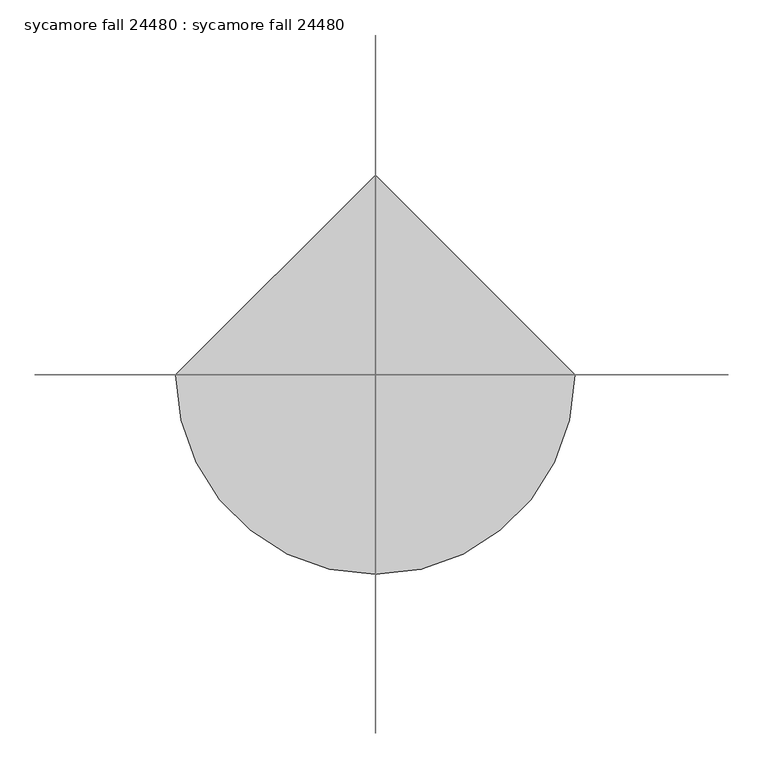
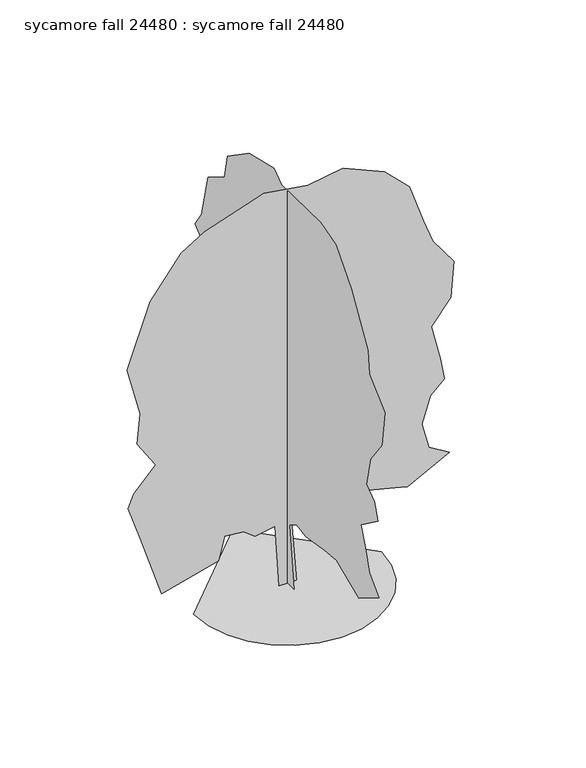
"""IFC4 building model written with IfcOpenShell, lengths in millimetres: proxy geometry, sycamore fall 24480 : sycamore fall 24480."""

from ifc_helpers import new_model, si_unit, origin, place, context, project, spatial, triangles, source, transform, mapped, element, save


def sycamore_fall_24480_sycamore_fall_24480_863b0ace(model_context):
    return source(origin(), model_context, "Body", "Tessellation", [
        triangles([(-350.832074, 1.54e-05, 0.0), (-519.2948653, -0.0002987, 2696.4612831), (-1365.6143188, -0.0002448, 2554.5769203), (-1847.3222706, -0.0002667, 2914.5200661), (-2641.8003754, -0.0002417, 2996.2572281), (-2887.1897575, -0.0001129, 2006.0772606), (-5273.8728561, 6.56e-05, 1384.1309212), (-6175.1399368, -0.000225, 4152.286084), (-6690.1497803, -0.000379, 5632.9271027), (-6446.9198593, -0.0004579, 6205.1631042), (-5531.3774872, -0.0006139, 7177.956633), (-6303.892543, -0.0007221, 8368.8851028), (-6175.1399368, -0.0008812, 9656.4100021), (-6722.3315369, -0.0011105, 11780.8123077), (-5756.700943, -0.001475, 14484.5891327), (-4453.1741135, -0.0017335, 16174.3476196), (-3471.3636932, -0.0018474, 16769.9263824), (-992.8925926, -0.0020555, 17606.8043701), (855.168877, -0.0021033, 17330.758429), (2322.4618732, -0.0021953, 17563.9046631), (4060.6175514, -0.0021804, 16802.108139), (5122.7937057, -0.0021041, 15772.114032), (5702.1926422, -0.001926, 14066.1495575), (6088.4498795, -0.0018163, 13003.948114), (6966.9590469, -0.0017145, 11827.7524658), (6860.9393555, -0.0015239, 10267.9906952), (6024.0607864, -0.0013645, 9237.9704269), (6413.7730453, -0.0011987, 7703.5832703), (6571.2529678, -0.001093, 6759.4920593), (5991.8790298, -0.0010025, 6212.3004593), (5637.8035492, -0.0008488, 5053.5531647), (5937.4468872, -0.0007297, 3944.5144638), (6794.2137772, -0.0007034, 3409.5910103), (5026.248436, -0.000519, 2510.7060516), (4511.2385925, -0.0005118, 2639.4635994), (2708.7041405, -0.0004867, 3090.0846405), (1446.8942413, -0.0004051, 2868.0127304), (1099.3210527, -0.0003972, 2929.1502777), (154.8209641, -0.0004225, 3487.5940979), (137.7651375, -0.0003627, 2991.9900467), (374.3524406, -1.63e-05, 0.0005208), (-4.19e-05, -473.1532413, 0.279514), (8.81e-05, -141.9955024, 2641.8259552), (4.65e-05, -654.9917061, 2992.6504715), (-2.36e-05, -1329.4982094, 2853.8647568), (-0.0001766, -2695.3944878, 3090.3639839), (-0.0002449, -3548.3255653, 3170.8058762), (-0.0004512, -5206.0293228, 2478.7960808), (-0.0005787, -6654.4885849, 3380.0506622), (-0.0004837, -5946.3626221, 4055.9948685), (-0.0004302, -5656.6756531, 4989.4437057), (-0.0003796, -5334.781929, 5826.3222748), (-0.0004627, -6557.9433151, 6727.5893555), (-0.0004219, -6332.6198593, 7435.7153183), (-0.0003424, -5721.0391663, 7854.179892), (-0.0003333, -6010.7261353, 9141.6792114), (-0.0003897, -6847.6297028, 10268.2697479), (-0.0003651, -7072.9275787, 11845.4560364), (-0.0002032, -5962.313974, 12858.9395233), (-0.0001885, -5849.7917725, 13873.2880737), (1.85e-05, -4658.8377228, 15836.7565979), (0.0001585, -3532.2727661, 17124.2814972), (0.0002908, -2408.9233109, 17446.1502228), (0.0005846, 426.8338666, 17381.7867096), (0.0006611, 989.4941082, 17779.9821716), (0.0008252, 2804.4619583, 17349.5793732), (0.0009496, 4340.6016243, 16287.3779297), (0.0009476, 4571.5633987, 15221.4429932), (0.0010368, 5770.0105957, 14484.8681854), (0.0010426, 6252.8386826, 12553.6069977), (0.0010659, 6703.459433, 11845.4560364), (0.0009883, 6168.8153229, 11394.8347046), (0.0009238, 6156.2678329, 9141.6792114), (0.0009203, 6220.656926, 8208.2303741), (0.0008056, 5448.1418701, 7146.0289307), (0.0008789, 6510.3433136, 6180.3977554), (0.0008979, 6703.459433, 5633.2061554), (0.0007283, 6027.5152267, 3219.1165901), (0.0006596, 5350.1995926, 2324.727578), (0.000618, 5264.7798065, 1458.5579189), (0.0004531, 3484.6733459, 1835.0388634), (0.0003699, 2840.9361855, 2156.9174721), (0.0003995, 2647.7947769, 3026.0004707), (0.0002502, 1392.4722725, 2446.6093826), (0.0002126, 1108.5996288, 2659.9106071), (0.0001468, 456.7626357, 2595.6741211), (6.52e-05, 395.9170037, 0.2796182), (-3939.7900429, -8e-07, 0.2427224), (-3835.6501785, -902.7404646, 0.2426104), (-3539.0037506, -1731.7626091, 0.2424986), (-3073.6507599, -2463.3147583, 0.2423909), (-2463.3147583, -3073.6507599, 0.2422916), (-1731.7626091, -3539.0037506, 0.242204), (-902.7404646, -3835.6501785, 0.2421326), (0.0001865, -3939.7900429, 0.2420805), (902.7404646, -3835.6501785, 0.2426061), (1731.7626091, -3539.0037506, 0.2426053), (2463.3147583, -3073.6507599, 0.2426287), (3073.6507599, -2463.3147583, 0.2426749), (3539.0037506, -1731.7626091, 0.2427417), (3835.6501785, -902.7404646, 0.2428276), (3939.7900429, 0.0003444, 0.242378), (-0.0005051, 3939.7900429, 0.2424674)], [[32, 33, 34], [41, 1, 2], [40, 41, 2], [6, 7, 8], [5, 6, 8], [32, 34, 35], [39, 40, 2], [31, 32, 35], [31, 35, 36], [28, 29, 30], [5, 8, 9], [5, 9, 10], [5, 10, 11], [4, 5, 11], [2, 3, 4], [39, 2, 4], [39, 4, 11], [24, 25, 26], [24, 26, 27], [30, 31, 36], [11, 12, 13], [39, 11, 13], [13, 14, 15], [39, 13, 15], [39, 15, 16], [39, 16, 17], [39, 17, 18], [39, 18, 19], [39, 19, 20], [39, 20, 21], [39, 21, 22], [39, 22, 23], [39, 23, 24], [39, 24, 27], [39, 27, 28], [39, 28, 30], [39, 30, 36], [39, 36, 37], [38, 39, 37], [48, 49, 50], [79, 80, 81], [86, 87, 42], [86, 42, 43], [47, 48, 50], [47, 50, 51], [70, 71, 72], [52, 53, 54], [52, 54, 55], [47, 51, 52], [83, 84, 85], [57, 58, 59], [56, 57, 59], [81, 82, 83], [79, 81, 83], [78, 79, 83], [77, 78, 83], [76, 77, 83], [75, 76, 83], [46, 47, 52], [64, 65, 66], [68, 69, 70], [66, 67, 68], [64, 66, 68], [75, 83, 85], [75, 85, 86], [75, 86, 43], [75, 43, 44], [73, 74, 75], [68, 70, 72], [64, 68, 72], [63, 64, 72], [63, 72, 73], [63, 73, 75], [63, 75, 44], [62, 63, 44], [61, 62, 44], [60, 61, 44], [59, 60, 44], [56, 59, 44], [55, 56, 44], [52, 55, 44], [46, 52, 44], [45, 46, 44], [102, 103, 88], [101, 102, 88], [101, 88, 89], [100, 101, 89], [100, 89, 90], [100, 90, 91], [99, 100, 91], [98, 99, 91], [98, 91, 92], [98, 92, 93], [98, 93, 94], [98, 94, 95], [98, 95, 96], [98, 96, 97]], closed=False),
    ])


if __name__ == "__main__":
    model = new_model("IFC4")
    model_context = context("Model", 3, world=origin())
    ifc_project = project(units=[si_unit("LENGTHUNIT", "METRE", prefix="MILLI")], contexts=[model_context])
    site = spatial("IfcSite", under=ifc_project)
    building = spatial("IfcBuilding", under=site)
    placement = place(None, origin())
    sycamore_fall_24480_sycamore_fall_24480_shape = sycamore_fall_24480_sycamore_fall_24480_863b0ace(model_context)
    element("IfcBuildingElementProxy", 1, Name="sycamore fall 24480 : sycamore fall 24480", ObjectType="sycamore fall 24480 : sycamore fall 24480", at=placement, inside=building, context=model_context, shape_type="MappedRepresentation", body=[
        mapped(sycamore_fall_24480_sycamore_fall_24480_shape, transform((0.0, 0.0, 0.0), x_axis=(1.0, 0.0, 0.0), y_axis=(0.0, 1.0, 0.0), z_axis=(0.0, 0.0, 1.0))),
    ])
    save(model, "model.ifc")

# Revit data of these elements
# Type "sycamore fall 24480 : sycamore fall 24480"
#   built-in parameter 1005195 = "RPC-16-G0VS-NDQ0-MUDG-8000-ST1L-LVER-AU"
#   Height = 0
